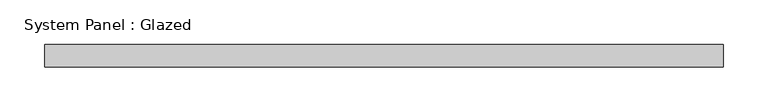
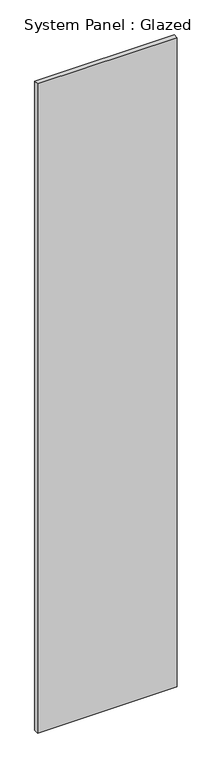
"""IFC4 building model written with IfcOpenShell, lengths in millimetres: plate geometry, System Panel : Glazed."""

from ifc_helpers import new_model, si_unit, origin, origin_with_axes, place, context, project, spatial, polyline, outline, extrude, source, transform, mapped, element, save


def system_panel_glazed_7e289b92(model_context):
    return source(origin(), model_context, "Body", "SweptSolid", [
        extrude(outline(polyline([(381.0, 19.05), (-381.0, 19.05), (-381.0, 44.45), (381.0, 44.45), (381.0, 19.05)])), origin_with_axes(), (0.0, 0.0, 1.0), 3746.5),
    ])


if __name__ == "__main__":
    model = new_model("IFC4")
    model_context = context("Model", 3, world=origin())
    ifc_project = project(units=[si_unit("LENGTHUNIT", "METRE", prefix="MILLI")], contexts=[model_context])
    site = spatial("IfcSite", under=ifc_project)
    building = spatial("IfcBuilding", under=site)
    placement = place(None, origin())
    system_panel_glazed_shape = system_panel_glazed_7e289b92(model_context)
    element("IfcPlate", 1, ObjectType="System Panel : Glazed", at=placement, inside=building, context=model_context, shape_type="MappedRepresentation", body=[
        mapped(system_panel_glazed_shape, transform((0.0, 0.0, 0.0), x_axis=(1.0, 0.0, 0.0), y_axis=(0.0, 1.0, 0.0), z_axis=(0.0, 0.0, 1.0))),
    ])
    save(model, "model.ifc")

# Revit data of these elements
# Type "System Panel : Glazed"
#   Construction Type Id = "GSP4R"
#   Analytic Construction = "1/8 in Pilkington single glazing"
#   Visual Light Transmittance = 0.9
#   Solar Heat Gain Coefficient = 0.86
#   Heat Transfer Coefficient (U) = 1.18115 BTU/(h·ft²·°F)
#   Define Thermal Properties by = 1
# Element 1 (IfcPlate, "System Panel : Glazed")
#   Materials on its faces: "Glass"
# Materials
#   "Glass": class "Glass", colour RGB 0 128 192, transparency 0.75, Description = "Soda Lime Glass", Cost = 0
